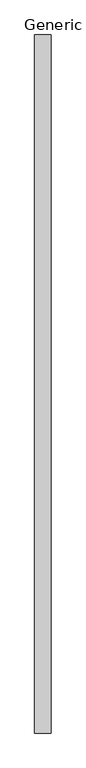
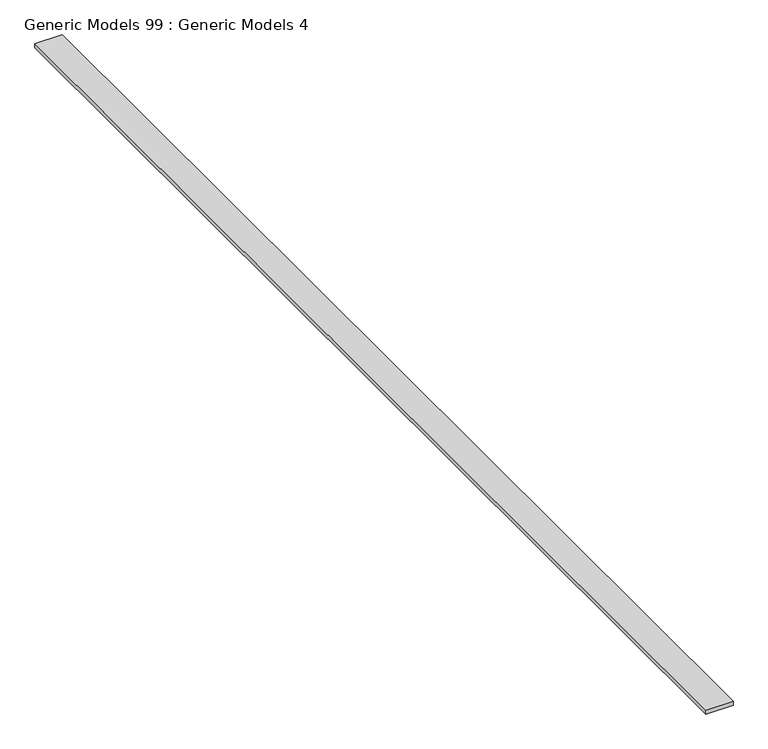
"""IFC4 building model written with IfcOpenShell, lengths in millimetres: proxy geometry, Generic Models 99 : Generic Models 4."""

from ifc_helpers import new_model, si_unit, frame, origin, place, context, project, spatial, polyline, outline, extrude, source, transform, mapped, element, save


def generic_models_99_generic_models_4_cf57d702(model_context):
    return source(origin(), model_context, "Body", "SweptSolid", [
        extrude(outline(polyline([(-5127.7986296, -464.1230338), (-5311.9486296, -464.1230338), (-5311.9486296, 7422.5769662), (-5127.7986296, 7422.5769662), (-5127.7986296, -464.1230338)])), frame((0.0, 0.0, 126736.221), z_axis=(0.0, 0.0, 1.0), x_axis=(1.0, 0.0, 0.0)), (0.0, 0.0, 1.0), 28.575),
    ])


if __name__ == "__main__":
    model = new_model("IFC4")
    model_context = context("Model", 3, world=origin())
    ifc_project = project(units=[si_unit("LENGTHUNIT", "METRE", prefix="MILLI")], contexts=[model_context])
    site = spatial("IfcSite", under=ifc_project)
    building = spatial("IfcBuilding", under=site)
    placement = place(None, origin())
    generic_models_99_generic_models_4_shape = generic_models_99_generic_models_4_cf57d702(model_context)
    element("IfcBuildingElementProxy", 1, Name="Generic Models 99 : Generic Models 4", ObjectType="Generic Models 99 : Generic Models 4", at=placement, inside=building, context=model_context, shape_type="MappedRepresentation", body=[
        mapped(generic_models_99_generic_models_4_shape, transform((0.0, 0.0, 0.0), x_axis=(1.0, 0.0, 0.0), y_axis=(0.0, 1.0, 0.0), z_axis=(0.0, 0.0, 1.0))),
    ])
    save(model, "model.ifc")

# Revit data of these elements
# Element 1 (IfcBuildingElementProxy, "Generic Models 99 : Generic Models 4")
#   Materials on its faces: "_2X BLOCKING AS REQUIRED"
# Materials
#   "_2X BLOCKING AS REQUIRED": class "Generic", colour RGB 177 130 114, transparency 0, Cost = 0
